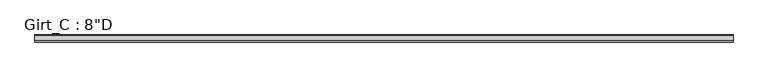
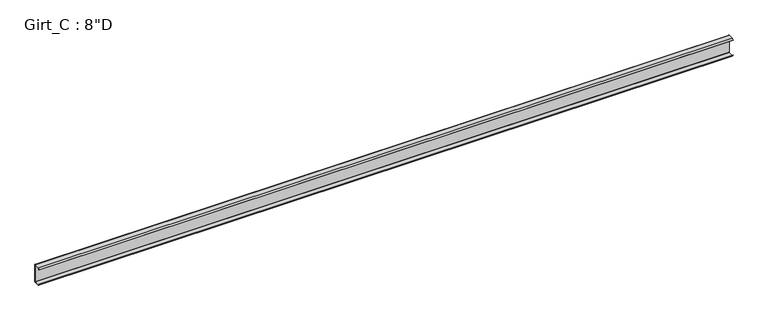
"""IFC4 building model written with IfcOpenShell, lengths in millimetres: beam geometry."""

from ifc_helpers import new_model, si_unit, point, frame, frame_2d, origin, place, context, project, spatial, polyline, circle_curve, trimmed, segment, composite_curve, outline, extrude, source, transform, mapped, element, save


def beam_0bb4d1e4(model_context):
    return source(origin(), model_context, "Body", "SweptSolid", [
        extrude(outline(composite_curve([segment(polyline([(-63.5, 101.6), (-3.3734375, 101.6)]), True, "CONTINUOUS"), segment(trimmed(circle_curve(frame_2d((-3.3734375, 96.8375)), 4.7625), [point((-3.3734375, 101.6))], [point((1.3890625, 96.8375))], False, "CARTESIAN"), True, "CONTINUOUS"), segment(polyline([(1.3890625, 96.8375), (1.3890625, -96.8375)]), True, "CONTINUOUS"), segment(trimmed(circle_curve(frame_2d((-3.3734375, -96.8375)), 4.7625), [point((1.3890625, -96.8375))], [point((-3.3734375, -101.6))], False, "CARTESIAN"), True, "CONTINUOUS"), segment(polyline([(-3.3734375, -101.6), (-63.5, -101.6), (-75.745104, -87.0068534), (-73.6169367, -85.221109), (-62.204539, -98.821875), (-3.2694106, -98.821875)]), True, "CONTINUOUS"), segment(trimmed(circle_curve(frame_2d((-3.3748024, -96.8389339)), 1.9857399), [point((-3.2694106, -98.821875))], [point((-1.3890625, -96.8389339))], True, "CARTESIAN"), True, "CONTINUOUS"), segment(polyline([(-1.3890625, -96.8389339), (-1.3890625, 96.8381931)]), True, "CONTINUOUS"), segment(trimmed(circle_curve(frame_2d((-3.3741066, 96.8381931)), 1.9850441), [point((-1.3890625, 96.8381931))], [point((-3.3005807, 98.821875))], True, "CARTESIAN"), True, "CONTINUOUS"), segment(polyline([(-3.3005807, 98.821875), (-62.204539, 98.821875), (-73.6169367, 85.221109), (-75.745104, 87.0068534), (-63.5, 101.6)]), True, "CONTINUOUS")], self_intersect=False)), frame((-3692.525, 0.0, 0.0), z_axis=(1.0, 0.0, 0.0), x_axis=(0.0, 1.0, 0.0)), (0.0, 0.0, 1.0), 7540.625),
    ])


if __name__ == "__main__":
    model = new_model("IFC4")
    model_context = context("Model", 3, world=origin())
    ifc_project = project(units=[si_unit("LENGTHUNIT", "METRE", prefix="MILLI")], contexts=[model_context])
    site = spatial("IfcSite", under=ifc_project)
    building = spatial("IfcBuilding", under=site)
    placement = place(None, origin())
    beam_shape = beam_0bb4d1e4(model_context)
    element("IfcBeam", 1, ObjectType="Girt_C : 8\"D", at=placement, inside=building, context=model_context, shape_type="MappedRepresentation", body=[
        mapped(beam_shape, transform((0.0, 0.0, 0.0), x_axis=(1.0, 0.0, 0.0), y_axis=(0.0, 1.0, 0.0), z_axis=(0.0, 0.0, 1.0))),
    ])
    save(model, "model.ifc")

# Revit data of these elements
# Type "Girt_C : 8\"D"
#   Web_Thickness = 0' - 0 7/64"
#   Length [instance default] = 10' - 0"
#   Leg_1 = 0' - 2 1/2"
#   Height = 0' - 8"
#   Structural Material [instance default] = none
# Element 1 (IfcBeam, "Girt_C : 8\"D")
#   Structural Material = Steel
#   Materials on its faces: "Steel"
# Materials
#   "Steel": class "Metal", colour RGB 118 118 114, transparency 0, Description = "Steel, mill finish", Cost = 0
